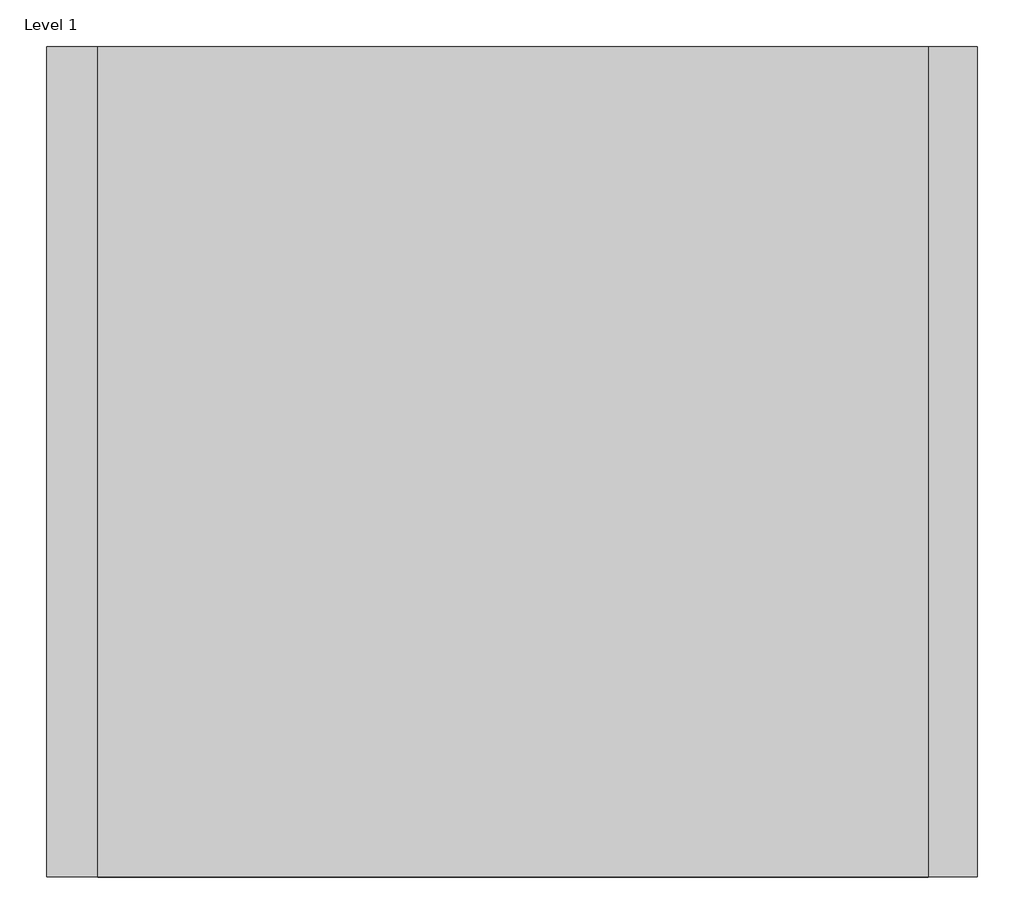
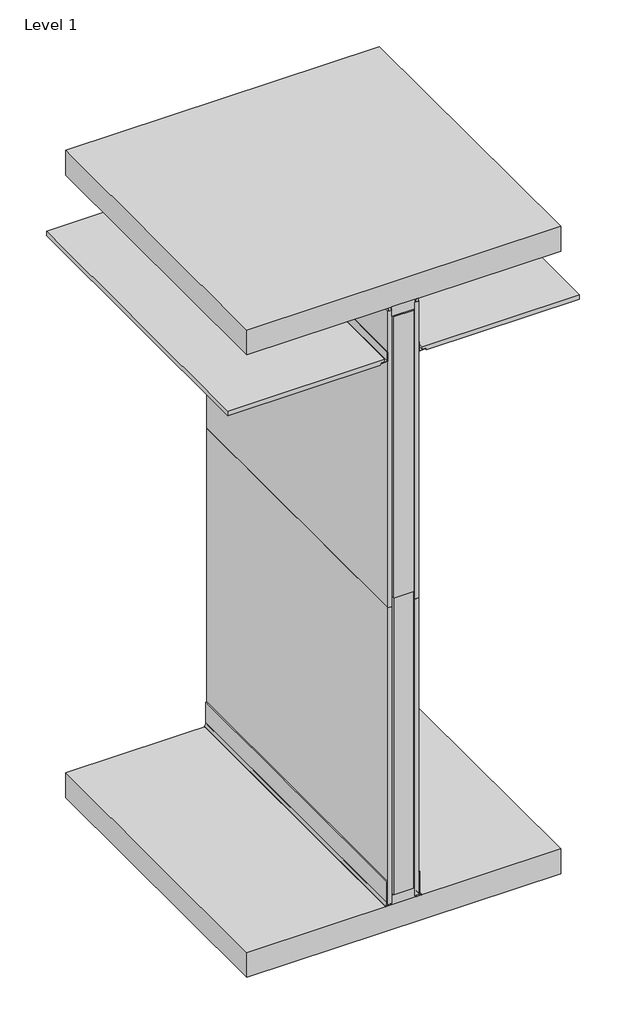
# One storey: 25 proxies.
"""IFC4 building model written with IfcOpenShell, lengths in millimetres."""

import ifcopenshell
import ifcopenshell.guid

model = None  # the IFC model being written
_history = None  # IfcOwnerHistory: only IFC2X3 demands one
_inside = {}  # id of a spatial element -> (the spatial element, [elements in it])
_under = {}  # id of a project, library or spatial element -> (it, [spatial elements below it])
_declared = {}  # id of a project -> (the project, [libraries it declares])
_typed = {}  # id of a type object -> (the type object, [elements of that type])
_made_of = {}  # id of a material, layer set ... -> (it, [elements and type objects made of it])


def new_model(schema):
    """Start an empty IFC model of exactly this schema.

    Asked for "IFC4X3", IfcOpenShell would pick the latest addendum, in which some entities
    have other attributes; the version numbers below select the first issue.
    IFC2X3 requires an IfcOwnerHistory on every rooted entity: one is made here for all.
    """
    global model, _history
    if schema == "IFC4X3":
        model = ifcopenshell.file(schema_version=(4, 3, 0, 0))
    else:
        model = ifcopenshell.file(schema=schema)
    _inside.clear()
    _under.clear()
    _declared.clear()
    _typed.clear()
    _made_of.clear()
    _history = None
    if model.schema == "IFC2X3":
        org = make("IfcOrganization", Name="unknown")
        user = make(
            "IfcPersonAndOrganization",
            ThePerson=make("IfcPerson", FamilyName="unknown"),
            TheOrganization=org,
        )
        app = make(
            "IfcApplication",
            ApplicationDeveloper=org,
            Version="unknown",
            ApplicationFullName="unknown",
            ApplicationIdentifier="unknown",
        )
        _history = make(
            "IfcOwnerHistory",
            OwningUser=user,
            OwningApplication=app,
            ChangeAction="ADDED",
            CreationDate=0,
        )
    return model


def make(cls, **values):
    """One entity of the class cls with the attributes given. An attribute that is None is left unset."""
    return model.create_entity(
        cls, **{name: value for name, value in values.items() if value is not None}
    )


def rooted(cls, **values):
    """An entity with a GlobalId (a new one), such as an element, a storey or a relation."""
    return make(cls, GlobalId=ifcopenshell.guid.new(), OwnerHistory=_history, **values)


def si_unit(unit_type, name, prefix=None):
    """IfcSIUnit, for example si_unit("LENGTHUNIT", "METRE", prefix="MILLI")."""
    return make("IfcSIUnit", UnitType=unit_type, Prefix=prefix, Name=name)


def assignment(units):
    """IfcUnitAssignment: the units of a project."""
    return None if units is None else make("IfcUnitAssignment", Units=units)


def point(xyz):
    """IfcCartesianPoint."""
    return None if xyz is None else make("IfcCartesianPoint", Coordinates=xyz)


def direction(xyz):
    """IfcDirection."""
    return None if xyz is None else make("IfcDirection", DirectionRatios=xyz)


def frame(location, z_axis=None, x_axis=None):
    """IfcAxis2Placement3D, a coordinate frame: its origin and axes. An axis left out is left unset."""
    return make(
        "IfcAxis2Placement3D",
        Location=point(location),
        Axis=direction(z_axis),
        RefDirection=direction(x_axis),
    )


def frame_2d(location, x_axis=None):
    """IfcAxis2Placement2D, a coordinate frame in the plane: its origin and x axis."""
    return make(
        "IfcAxis2Placement2D", Location=point(location), RefDirection=direction(x_axis)
    )


def origin():
    """The frame at (0, 0, 0) with its axes left unset."""
    return frame((0.0, 0.0, 0.0))


def place(relative_to, where):
    """IfcLocalPlacement: puts the frame where relative to a parent placement (None: the world)."""
    return make(
        "IfcLocalPlacement", PlacementRelTo=relative_to, RelativePlacement=where
    )


def context(
    kind, dimensions, precision=None, world=None, true_north=None, identifier=None
):
    """IfcGeometricRepresentationContext, for example the 3D "Model" context."""
    return make(
        "IfcGeometricRepresentationContext",
        ContextIdentifier=identifier,
        ContextType=kind,
        CoordinateSpaceDimension=dimensions,
        Precision=precision,
        WorldCoordinateSystem=world,
        TrueNorth=true_north,
    )


def project(units=None, contexts=None):
    """IfcProject with its units and contexts."""
    return rooted(
        "IfcProject",
        Name="project",
        RepresentationContexts=contexts,
        UnitsInContext=assignment(units),
    )


def spatial(cls, under=None, at=None, **own):
    """A site, building, storey or space (cls), placed at a placement, below another one or the project."""
    s = rooted(cls, ObjectPlacement=at, **own)
    if under is not None:
        _under.setdefault(under.id(), (under, []))[1].append(s)
    return s


def polyline(points):
    """IfcPolyline through the points."""
    return make("IfcPolyline", Points=[point(p) for p in points])


def circle_curve(where, radius):
    """IfcCircle in the frame where."""
    return make("IfcCircle", Position=where, Radius=radius)


def trimmed(basis, trim1, trim2, sense, master):
    """IfcTrimmedCurve: the piece of a basis curve between two trims."""
    return make(
        "IfcTrimmedCurve",
        BasisCurve=basis,
        Trim1=trim1,
        Trim2=trim2,
        SenseAgreement=sense,
        MasterRepresentation=master,
    )


def segment(curve, same_sense, transition):
    """IfcCompositeCurveSegment."""
    return make(
        "IfcCompositeCurveSegment",
        Transition=transition,
        SameSense=same_sense,
        ParentCurve=curve,
    )


def composite_curve(segments, self_intersect=None):
    """IfcCompositeCurve: segments joined end to end."""
    return make("IfcCompositeCurve", Segments=segments, SelfIntersect=self_intersect)


def outline(outer, holes=None, kind="AREA"):
    """IfcArbitraryClosedProfileDef: a profile drawn as a closed curve; with holes, ...WithVoids."""
    if holes is None:
        return make("IfcArbitraryClosedProfileDef", ProfileType=kind, OuterCurve=outer)
    return make(
        "IfcArbitraryProfileDefWithVoids",
        ProfileType=kind,
        OuterCurve=outer,
        InnerCurves=holes,
    )


def extrude(swept, where, along, depth):
    """IfcExtrudedAreaSolid: the profile swept, set in the frame where, extruded along a direction by depth."""
    return make(
        "IfcExtrudedAreaSolid",
        SweptArea=swept,
        Position=where,
        ExtrudedDirection=direction(along),
        Depth=depth,
    )


def shape(context_of_items, identifier, shape_type, items):
    """IfcShapeRepresentation: the items that make up one representation, for example the "Body"."""
    return make(
        "IfcShapeRepresentation",
        ContextOfItems=context_of_items,
        RepresentationIdentifier=identifier,
        RepresentationType=shape_type,
        Items=items,
    )


def source(mapping_origin, context_of_items, identifier, shape_type, items):
    """IfcRepresentationMap: a shape defined once, which mapped items show again and again."""
    return make(
        "IfcRepresentationMap",
        MappingOrigin=mapping_origin,
        MappedRepresentation=shape(context_of_items, identifier, shape_type, items),
    )


def transform(
    local_origin,
    x_axis=None,
    y_axis=None,
    z_axis=None,
    scale=None,
    scale2=None,
    scale3=None,
    uniform=True,
):
    """IfcCartesianTransformationOperator3D, or its non-uniform kind. x_axis, y_axis, z_axis: its Axis1, 2, 3."""
    if uniform:
        return make(
            "IfcCartesianTransformationOperator3D",
            Axis1=direction(x_axis),
            Axis2=direction(y_axis),
            LocalOrigin=point(local_origin),
            Scale=scale,
            Axis3=direction(z_axis),
        )
    return make(
        "IfcCartesianTransformationOperator3DnonUniform",
        Axis1=direction(x_axis),
        Axis2=direction(y_axis),
        LocalOrigin=point(local_origin),
        Scale=scale,
        Axis3=direction(z_axis),
        Scale2=scale2,
        Scale3=scale3,
    )


def mapped(mapping_source, mapping_target):
    """IfcMappedItem: shows the shape of a source again, moved by a transform."""
    return make(
        "IfcMappedItem", MappingSource=mapping_source, MappingTarget=mapping_target
    )


def made_of(thing, what):
    """Note that an element or type object is made of a material, layer set ...; save() writes the relation."""
    if what is not None:
        _made_of.setdefault(what.id(), (what, []))[1].append(thing)
    return thing


def element(
    cls,
    number,
    at=None,
    inside=None,
    cuts=None,
    type_object=None,
    material=None,
    context=None,
    identifier="Body",
    shape_type=None,
    held_by="IfcProductDefinitionShape",
    body=None,
    shapes=None,
    **own,
):
    """One element of the class cls, such as IfcWall. Its Tag is "e" and its number.

    at: its placement. inside: the storey or other place that contains it. cuts: it is an
    opening in that element (IfcRelVoidsElement). A single representation is given by context,
    identifier, shape_type and body (its items); several are given by shapes. held_by: the class
    of the entity that holds the representations. save() writes the other relations.
    """
    e = rooted(cls, Tag="e%d" % number, ObjectPlacement=at, **own)
    if body is not None:
        shapes = [shape(context, identifier, shape_type, body)]
    if shapes is not None:
        e.Representation = make(held_by, Representations=shapes)
    if inside is not None:
        _inside.setdefault(inside.id(), (inside, []))[1].append(e)
    if cuts is not None:
        rooted(
            "IfcRelVoidsElement", RelatingBuildingElement=cuts, RelatedOpeningElement=e
        )
    if type_object is not None:
        _typed.setdefault(type_object.id(), (type_object, []))[1].append(e)
    return made_of(e, material)


def aggregate(whole, parts):
    """IfcRelAggregates: a whole, such as a stair, and the parts it consists of."""
    return rooted("IfcRelAggregates", RelatingObject=whole, RelatedObjects=parts)


def save(model, path):
    """Write the relations noted so far, then the file.

    IfcRelAggregates (storeys below a building ...), IfcRelContainedInSpatialStructure (elements
    in a storey), IfcRelDefinesByType, IfcRelAssociatesMaterial and IfcRelDeclares: one each for
    every whole, place, type object, material and project.
    """
    for whole, parts in _under.values():
        aggregate(whole, parts)
    for where, things in _inside.values():
        rooted(
            "IfcRelContainedInSpatialStructure",
            RelatedElements=things,
            RelatingStructure=where,
        )
    for kind, things in _typed.values():
        rooted("IfcRelDefinesByType", RelatedObjects=things, RelatingType=kind)
    for what, things in _made_of.values():
        rooted("IfcRelAssociatesMaterial", RelatedObjects=things, RelatingMaterial=what)
    for by, libraries in _declared.values():
        rooted("IfcRelDeclares", RelatingContext=by, RelatedDefinitions=libraries)
    model.write(path)


def generic_models_70_generic_models_1_2fc778b0(model_context):
    return source(origin(), model_context, "Body", "SweptSolid", [
        extrude(outline(polyline([(51059.1296235, 0.0), (51043.2546235, 0.0), (51043.2546235, 1219.2), (51059.1296235, 1219.2), (51059.1296235, 0.0)])), frame((0.0, 0.0, 34.479891), z_axis=(0.0, 0.0, 1.0), x_axis=(1.0, 0.0, 0.0)), (0.0, 0.0, 1.0), 1219.2),
    ])


def generic_models_71_generic_models_1_dfea5cc7(model_context):
    return source(origin(), model_context, "Body", "SweptSolid", [
        extrude(outline(composite_curve([segment(trimmed(circle_curve(frame_2d((31.025412, 51021.9897405)), 4.3100275), [point((27.850412, 51019.075))], [point((34.200412, 51019.075))], True, "CARTESIAN"), True, "CONTINUOUS"), segment(polyline([(34.200412, 51019.075), (34.200412, 51009.55)]), True, "CONTINUOUS"), segment(trimmed(circle_curve(frame_2d((31.025412, 51012.4647405)), 4.3100275), [point((34.200412, 51009.55))], [point((27.850412, 51009.55))], False, "CARTESIAN"), True, "CONTINUOUS"), segment(polyline([(27.850412, 51009.55), (27.850412, 51019.075)]), True, "CONTINUOUS")], self_intersect=False)), frame((0.0, 0.0, 0.0), z_axis=(0.0, 1.0, 0.0), x_axis=(0.0, 0.0, 1.0)), (0.0, 0.0, 1.0), 1219.2),
    ])


def generic_models_72_generic_models_1_f511e09d(model_context):
    return source(origin(), model_context, "Body", "SweptSolid", [
        extrude(outline(polyline([(48561.625, 592.1375), (48472.725, 592.1375), (48472.725, 630.2375), (48561.625, 630.2375), (48561.625, 592.1375)])), frame((0.0, 0.0, 65.950412), z_axis=(0.0, 0.0, 1.0), x_axis=(1.0, 0.0, 0.0)), (0.0, 0.0, 1.0), 2381.25),
    ])


def generic_models_73_generic_models_1_7c4ccb31(model_context):
    return source(origin(), model_context, "Body", "SweptSolid", [
        extrude(outline(composite_curve([segment(polyline([(101.6, 51108.5310187), (15.4496307, 51108.5310187)]), True, "CONTINUOUS"), segment(trimmed(circle_curve(frame_2d((15.4496307, 51126.3707155)), 17.8396968), [point((15.4496307, 51108.5310187))], [point((0.0, 51117.4508671))], False, "CARTESIAN"), True, "CONTINUOUS"), segment(polyline([(0.0, 51117.4508671), (2.7496307, 51119.0383671)]), True, "CONTINUOUS"), segment(trimmed(circle_curve(frame_2d((15.4496307, 51126.3707155)), 14.6646968), [point((2.7496307, 51119.0383671))], [point((15.4496307, 51111.7060187))], True, "CARTESIAN"), True, "CONTINUOUS"), segment(polyline([(15.4496307, 51111.7060187), (99.5131982, 51111.7060187)]), True, "CONTINUOUS"), segment(trimmed(circle_curve(frame_2d((99.5131982, 51109.6192169)), 2.0868018), [point((99.5131982, 51111.7060187))], [point((101.6, 51109.6192169))], False, "CARTESIAN"), True, "CONTINUOUS"), segment(polyline([(101.6, 51109.6192169), (101.6, 51108.5310187)]), True, "CONTINUOUS")], self_intersect=False)), frame((0.0, 0.0, 0.0), z_axis=(0.0, 1.0, 0.0), x_axis=(0.0, 0.0, 1.0)), (0.0, 0.0, 1.0), 1219.2),
    ])


def generic_models_74_generic_models_1_1398e35e(model_context):
    return source(origin(), model_context, "Body", "SweptSolid", [
        extrude(outline(polyline([(48561.625, 0.0), (48472.725, 0.0), (48472.725, 1219.2), (48561.625, 1219.2), (48561.625, 0.0)])), frame((0.0, 0.0, 2447.200412), z_axis=(0.0, 0.0, 1.0), x_axis=(1.0, 0.0, 0.0)), (0.0, 0.0, 1.0), 38.1),
    ])


def generic_models_75_generic_models_1_c604be2e(model_context):
    return source(origin(), model_context, "Body", "SweptSolid", [
        extrude(outline(composite_curve([segment(trimmed(circle_curve(frame_2d((2472.600412, 51037.604481)), 8.620055), [point((2466.250412, 51031.775))], [point((2478.950412, 51031.775))], True, "CARTESIAN"), True, "CONTINUOUS"), segment(polyline([(2478.950412, 51031.775), (2478.950412, 51022.25)]), True, "CONTINUOUS"), segment(trimmed(circle_curve(frame_2d((2472.600412, 51028.079481)), 8.620055), [point((2478.950412, 51022.25))], [point((2466.250412, 51022.25))], False, "CARTESIAN"), True, "CONTINUOUS"), segment(polyline([(2466.250412, 51022.25), (2466.250412, 51031.775)]), True, "CONTINUOUS")], self_intersect=False)), frame((0.0, 0.0, 0.0), z_axis=(0.0, 1.0, 0.0), x_axis=(0.0, 0.0, 1.0)), (0.0, 0.0, 1.0), 1219.2),
    ])


def generic_models_77_generic_models_1_8544dbac(model_context):
    return source(origin(), model_context, "Body", "SweptSolid", [
        extrude(outline(polyline([(49128.3625, 0.0), (47909.1625, 0.0), (47909.1625, 1219.2), (49128.3625, 1219.2), (49128.3625, 0.0)])), frame((0.0, 0.0, 2485.300412), z_axis=(0.0, 0.0, 1.0), x_axis=(1.0, 0.0, 0.0)), (0.0, 0.0, 1.0), 101.6),
    ])


def generic_models_78_generic_models_1_faebf22d(model_context):
    return source(origin(), model_context, "Body", "SweptSolid", [
        extrude(outline(polyline([(51649.6572697, 0.0), (50430.4572697, 0.0), (50430.4572697, 1219.2), (51649.6572697, 1219.2), (51649.6572697, 0.0)])), frame((0.0, 0.0, -73.749588), z_axis=(0.0, 0.0, 1.0), x_axis=(1.0, 0.0, 0.0)), (0.0, 0.0, 1.0), 101.6),
    ])


def generic_models_79_generic_models_1_6d14886f(model_context):
    return source(origin(), model_context, "Body", "SweptSolid", [
        extrude(outline(polyline([(49776.0625, 0.0), (49699.8625, 0.0), (49699.8625, 1219.2), (49776.0625, 1219.2), (49776.0625, 0.0)])), frame((0.0, 0.0, 29.437912), z_axis=(0.0, 0.0, 1.0), x_axis=(1.0, 0.0, 0.0)), (0.0, 0.0, 1.0), 1219.2),
    ])


def generic_models_80_generic_models_1_8b1a960f(model_context):
    return source(origin(), model_context, "Body", "SweptSolid", [
        extrude(outline(polyline([(48556.8625, 0.0), (48480.6625, 0.0), (48480.6625, 1219.2), (48556.8625, 1219.2), (48556.8625, 0.0)])), frame((0.0, 0.0, 1264.512912), z_axis=(0.0, 0.0, 1.0), x_axis=(1.0, 0.0, 0.0)), (0.0, 0.0, 1.0), 1219.2),
    ])


def generic_models_81_generic_models_1_62cb9d11(model_context):
    return source(origin(), model_context, "Body", "SweptSolid", [
        extrude(outline(polyline([(2304.9709098, 49799.875), (2266.8709098, 49799.875), (2266.8709098, 49825.275), (2268.4584098, 49825.275), (2268.4584098, 49801.4625), (2304.9709098, 49801.4625), (2304.9709098, 49799.875)])), frame((0.0, 0.0, 0.0), z_axis=(0.0, 1.0, 0.0), x_axis=(0.0, 0.0, 1.0)), (0.0, 0.0, 1.0), 1219.2),
    ])


def generic_models_82_generic_models_1_f14c7ad8(model_context):
    return source(origin(), model_context, "Body", "SweptSolid", [
        extrude(outline(polyline([(2442.2225782, 49800.66875), (2442.2225782, 49799.875), (2439.6727146, 49799.875), (2437.6759782, 49723.675), (2435.6792418, 49799.875), (2433.1293782, 49799.875), (2433.1293782, 49800.66875), (2442.2225782, 49800.66875)])), frame((0.0, 565.15, 0.0), z_axis=(0.0, 1.0, 0.0), x_axis=(0.0, 0.0, 1.0)), (0.0, 0.0, 1.0), 12.7),
    ])


def generic_models_83_generic_models_1_66a13d42(model_context):
    return source(origin(), model_context, "Body", "SweptSolid", [
        extrude(outline(polyline([(2457.6119589, 49845.474547), (2457.6119589, 49854.567747), (2458.4057089, 49854.567747), (2458.4057089, 49852.0178834), (2534.6057089, 49850.021147), (2458.4057089, 49848.0244106), (2458.4057089, 49845.474547), (2457.6119589, 49845.474547)])), frame((0.0, 565.15, 0.0), z_axis=(0.0, 1.0, 0.0), x_axis=(0.0, 0.0, 1.0)), (0.0, 0.0, 1.0), 12.7),
    ])


def generic_models_84_generic_models_1_80fe95b7(model_context):
    return source(origin(), model_context, "Body", "SweptSolid", [
        extrude(outline(polyline([(48432.6703765, 0.0), (48416.7953765, 0.0), (48416.7953765, 1219.2), (48432.6703765, 1219.2), (48432.6703765, 0.0)])), frame((0.0, 0.0, 34.479891), z_axis=(0.0, 0.0, 1.0), x_axis=(1.0, 0.0, 0.0)), (0.0, 0.0, 1.0), 1219.2),
    ])


def generic_models_85_generic_models_1_c4fdf2dc(model_context):
    return source(origin(), model_context, "Body", "SweptSolid", [
        extrude(outline(composite_curve([segment(polyline([(27.850412, 48456.85), (27.850412, 48466.375)]), True, "CONTINUOUS"), segment(trimmed(circle_curve(frame_2d((31.025412, 48463.4602595)), 4.3100275), [point((27.850412, 48466.375))], [point((34.200412, 48466.375))], False, "CARTESIAN"), True, "CONTINUOUS"), segment(polyline([(34.200412, 48466.375), (34.200412, 48456.85)]), True, "CONTINUOUS"), segment(trimmed(circle_curve(frame_2d((31.025412, 48453.9352595)), 4.3100275), [point((34.200412, 48456.85))], [point((27.850412, 48456.85))], True, "CARTESIAN"), True, "CONTINUOUS")], self_intersect=False)), frame((0.0, 0.0, 0.0), z_axis=(0.0, 1.0, 0.0), x_axis=(0.0, 0.0, 1.0)), (0.0, 0.0, 1.0), 1219.2),
    ])


def generic_models_86_generic_models_1_e8e5dea3(model_context):
    return source(origin(), model_context, "Body", "SweptSolid", [
        extrude(outline(composite_curve([segment(polyline([(101.6, 48367.3939813), (101.6, 48366.3057831)]), True, "CONTINUOUS"), segment(trimmed(circle_curve(frame_2d((99.5131982, 48366.3057831)), 2.0868018), [point((101.6, 48366.3057831))], [point((99.5131982, 48364.2189813))], False, "CARTESIAN"), True, "CONTINUOUS"), segment(polyline([(99.5131982, 48364.2189813), (15.4496307, 48364.2189813)]), True, "CONTINUOUS"), segment(trimmed(circle_curve(frame_2d((15.4496307, 48349.5542845)), 14.6646968), [point((15.4496307, 48364.2189813))], [point((2.7496307, 48356.8866329))], True, "CARTESIAN"), True, "CONTINUOUS"), segment(polyline([(2.7496307, 48356.8866329), (0.0, 48358.4741329)]), True, "CONTINUOUS"), segment(trimmed(circle_curve(frame_2d((15.4496307, 48349.5542845)), 17.8396968), [point((0.0, 48358.4741329))], [point((15.4496307, 48367.3939813))], False, "CARTESIAN"), True, "CONTINUOUS"), segment(polyline([(15.4496307, 48367.3939813), (101.6, 48367.3939813)]), True, "CONTINUOUS")], self_intersect=False)), frame((0.0, 0.0, 0.0), z_axis=(0.0, 1.0, 0.0), x_axis=(0.0, 0.0, 1.0)), (0.0, 0.0, 1.0), 1219.2),
    ])


def generic_models_87_generic_models_1_0e45ed3c(model_context):
    return source(origin(), model_context, "Body", "SweptSolid", [
        extrude(outline(composite_curve([segment(polyline([(2466.250412, 48444.15), (2466.250412, 48453.675)]), True, "CONTINUOUS"), segment(trimmed(circle_curve(frame_2d((2472.600412, 48447.845519)), 8.620055), [point((2466.250412, 48453.675))], [point((2478.950412, 48453.675))], False, "CARTESIAN"), True, "CONTINUOUS"), segment(polyline([(2478.950412, 48453.675), (2478.950412, 48444.15)]), True, "CONTINUOUS"), segment(trimmed(circle_curve(frame_2d((2472.600412, 48438.320519)), 8.620055), [point((2478.950412, 48444.15))], [point((2466.250412, 48444.15))], True, "CARTESIAN"), True, "CONTINUOUS")], self_intersect=False)), frame((0.0, 0.0, 0.0), z_axis=(0.0, 1.0, 0.0), x_axis=(0.0, 0.0, 1.0)), (0.0, 0.0, 1.0), 1219.2),
    ])


def generic_models_89_generic_models_1_217c0eea(model_context):
    return source(origin(), model_context, "Body", "SweptSolid", [
        extrude(outline(polyline([(2304.9709098, 49676.05), (2304.9709098, 49674.4625), (2268.4584098, 49674.4625), (2268.4584098, 49650.65), (2266.8709098, 49650.65), (2266.8709098, 49676.05), (2304.9709098, 49676.05)])), frame((0.0, 0.0, 0.0), z_axis=(0.0, 1.0, 0.0), x_axis=(0.0, 0.0, 1.0)), (0.0, 0.0, 1.0), 1219.2),
    ])


def generic_models_90_generic_models_1_e41f1d4b(model_context):
    return source(origin(), model_context, "Body", "SweptSolid", [
        extrude(outline(polyline([(2281.1808399, 49662.5798593), (2281.1808399, 49052.9798593), (2262.1308399, 49052.9798593), (2262.1308399, 49646.9908455), (2270.0683399, 49649.8798593), (2270.0683399, 49662.5798593), (2281.1808399, 49662.5798593)])), frame((0.0, 0.0, 0.0), z_axis=(0.0, 1.0, 0.0), x_axis=(0.0, 0.0, 1.0)), (0.0, 0.0, 1.0), 1219.2),
    ])


def generic_models_91_generic_models_1_b13b52c1(model_context):
    return source(origin(), model_context, "Body", "SweptSolid", [
        extrude(outline(polyline([(2442.2225782, 49675.25625), (2433.1293782, 49675.25625), (2433.1293782, 49676.05), (2435.6792418, 49676.05), (2437.6759782, 49752.25), (2439.6727146, 49676.05), (2442.2225782, 49676.05), (2442.2225782, 49675.25625)])), frame((0.0, 565.15, 0.0), z_axis=(0.0, 1.0, 0.0), x_axis=(0.0, 0.0, 1.0)), (0.0, 0.0, 1.0), 12.7),
    ])


def generic_models_92_generic_models_1_05829357(model_context):
    return source(origin(), model_context, "Body", "SweptSolid", [
        extrude(outline(polyline([(67.537912, 48511.0409), (66.744162, 48511.0409), (66.744162, 48513.5907636), (-9.455838, 48515.5875), (66.744162, 48517.5842364), (66.744162, 48520.1341), (67.537912, 48520.1341), (67.537912, 48511.0409)])), frame((0.0, 565.15, 0.0), z_axis=(0.0, 1.0, 0.0), x_axis=(0.0, 0.0, 1.0)), (0.0, 0.0, 1.0), 12.7),
    ])


def generic_models_93_generic_models_1_4e4062ca(model_context):
    return source(origin(), model_context, "Body", "SweptSolid", [
        extrude(outline(polyline([(2281.1808399, 49813.3451407), (2270.0683399, 49813.3451407), (2270.0683399, 49826.0451407), (2262.1308399, 49828.9341545), (2262.1308399, 50422.9451407), (2281.1808399, 50422.9451407), (2281.1808399, 49813.3451407)])), frame((0.0, 0.0, 0.0), z_axis=(0.0, 1.0, 0.0), x_axis=(0.0, 0.0, 1.0)), (0.0, 0.0, 1.0), 1219.2),
    ])


model = new_model("IFC4")

# Units and contexts
model_context = context("Model", 3, world=origin())
ifc_project = project(units=[si_unit("LENGTHUNIT", "METRE", prefix="MILLI")], contexts=[model_context])

# Site, building, storey
site = spatial("IfcSite", under=ifc_project)
building = spatial("IfcBuilding", under=site)
storey = spatial("IfcBuildingStorey", under=building, Name="Level 1", Elevation=266395.2)

# Proxies
placement = place(None, origin())
generic_models_70_generic_models_1_shape = generic_models_70_generic_models_1_2fc778b0(model_context)
element("IfcBuildingElementProxy", 1, Name="Generic Models 70 : Generic Models 1", ObjectType="Generic Models 70 : Generic Models 1", at=placement, inside=storey, context=model_context, shape_type="MappedRepresentation", body=[
    mapped(generic_models_70_generic_models_1_shape, transform((-2481.6296235, 0.0, -0.279479), x_axis=(1.0, 0.0, 0.0), y_axis=(0.0, 1.0, 0.0), z_axis=(0.0, 0.0, 1.0))),
])
generic_models_71_generic_models_1_shape = generic_models_71_generic_models_1_dfea5cc7(model_context)
element("IfcBuildingElementProxy", 2, Name="Generic Models 71 : Generic Models 1", ObjectType="Generic Models 71 : Generic Models 1", at=placement, inside=storey, context=model_context, shape_type="MappedRepresentation", body=[
    mapped(generic_models_71_generic_models_1_shape, transform((-2441.575, 0.0, 0.0), x_axis=(1.0, 0.0, 0.0), y_axis=(0.0, 1.0, 0.0), z_axis=(0.0, 0.0, 1.0))),
])
generic_models_72_generic_models_1_shape = generic_models_72_generic_models_1_f511e09d(model_context)
element("IfcBuildingElementProxy", 3, Name="Generic Models 72 : Generic Models 1", ObjectType="Generic Models 72 : Generic Models 1", at=placement, inside=storey, context=model_context, shape_type="MappedRepresentation", body=[
    mapped(generic_models_72_generic_models_1_shape, transform((0.0, 0.0, 0.0), x_axis=(1.0, 0.0, 0.0), y_axis=(0.0, 1.0, 0.0), z_axis=(0.0, 0.0, 1.0))),
])
generic_models_73_generic_models_1_shape = generic_models_73_generic_models_1_7c4ccb31(model_context)
element("IfcBuildingElementProxy", 4, Name="Generic Models 73 : Generic Models 1", ObjectType="Generic Models 73 : Generic Models 1", at=placement, inside=storey, context=model_context, shape_type="MappedRepresentation", body=[
    mapped(generic_models_73_generic_models_1_shape, transform((-2531.0310187, 0.0, 27.850412), x_axis=(1.0, 0.0, 0.0), y_axis=(0.0, 1.0, 0.0), z_axis=(0.0, 0.0, 1.0))),
])
generic_models_74_generic_models_1_shape = generic_models_74_generic_models_1_1398e35e(model_context)
element("IfcBuildingElementProxy", 5, Name="Generic Models 74 : Generic Models 1", ObjectType="Generic Models 74 : Generic Models 1", at=placement, inside=storey, context=model_context, shape_type="MappedRepresentation", body=[
    mapped(generic_models_74_generic_models_1_shape, transform((0.0, 0.0, 0.0), x_axis=(1.0, 0.0, 0.0), y_axis=(0.0, 1.0, 0.0), z_axis=(0.0, 0.0, 1.0))),
])
generic_models_75_generic_models_1_shape = generic_models_75_generic_models_1_c604be2e(model_context)
element("IfcBuildingElementProxy", 6, Name="Generic Models 75 : Generic Models 1", ObjectType="Generic Models 75 : Generic Models 1", at=placement, inside=storey, context=model_context, shape_type="MappedRepresentation", body=[
    mapped(generic_models_75_generic_models_1_shape, transform((-2454.275, 0.0, 6.35), x_axis=(1.0, 0.0, 0.0), y_axis=(0.0, 1.0, 0.0), z_axis=(0.0, 0.0, 1.0))),
])
element("IfcBuildingElementProxy", 7, Name="Generic Models 76 : Generic Models 1", ObjectType="Generic Models 76 : Generic Models 1", at=placement, inside=storey, context=model_context, shape_type="MappedRepresentation", body=[
    mapped(generic_models_70_generic_models_1_shape, transform((-2481.6296235, 0.0, 1218.920521), x_axis=(1.0, 0.0, 0.0), y_axis=(0.0, 1.0, 0.0), z_axis=(0.0, 0.0, 1.0))),
])
generic_models_77_generic_models_1_shape = generic_models_77_generic_models_1_8544dbac(model_context)
element("IfcBuildingElementProxy", 8, Name="Generic Models 77 : Generic Models 1", ObjectType="Generic Models 77 : Generic Models 1", at=placement, inside=storey, context=model_context, shape_type="MappedRepresentation", body=[
    mapped(generic_models_77_generic_models_1_shape, transform((0.0, 0.0, 0.0), x_axis=(1.0, 0.0, 0.0), y_axis=(0.0, 1.0, 0.0), z_axis=(0.0, 0.0, 1.0))),
])
generic_models_78_generic_models_1_shape = generic_models_78_generic_models_1_faebf22d(model_context)
element("IfcBuildingElementProxy", 9, Name="Generic Models 78 : Generic Models 1", ObjectType="Generic Models 78 : Generic Models 1", at=placement, inside=storey, context=model_context, shape_type="MappedRepresentation", body=[
    mapped(generic_models_78_generic_models_1_shape, transform((-2521.2947697, 0.0, 0.0), x_axis=(1.0, 0.0, 0.0), y_axis=(0.0, 1.0, 0.0), z_axis=(0.0, 0.0, 1.0))),
])
generic_models_79_generic_models_1_shape = generic_models_79_generic_models_1_6d14886f(model_context)
element("IfcBuildingElementProxy", 10, Name="Generic Models 79 : Generic Models 1", ObjectType="Generic Models 79 : Generic Models 1", at=placement, inside=storey, context=model_context, shape_type="MappedRepresentation", body=[
    mapped(generic_models_79_generic_models_1_shape, transform((-1220.7875, 0.0, 36.5125), x_axis=(1.0, 0.0, 0.0), y_axis=(0.0, 1.0, 0.0), z_axis=(0.0, 0.0, 1.0))),
])
generic_models_80_generic_models_1_shape = generic_models_80_generic_models_1_8b1a960f(model_context)
element("IfcBuildingElementProxy", 11, Name="Generic Models 80 : Generic Models 1", ObjectType="Generic Models 80 : Generic Models 1", at=placement, inside=storey, context=model_context, shape_type="MappedRepresentation", body=[
    mapped(generic_models_80_generic_models_1_shape, transform((0.0, 0.0, -41.275), x_axis=(1.0, 0.0, 0.0), y_axis=(0.0, 1.0, 0.0), z_axis=(0.0, 0.0, 1.0))),
])
generic_models_81_generic_models_1_shape = generic_models_81_generic_models_1_62cb9d11(model_context)
element("IfcBuildingElementProxy", 12, Name="Generic Models 81 : Generic Models 1", ObjectType="Generic Models 81 : Generic Models 1", at=placement, inside=storey, context=model_context, shape_type="MappedRepresentation", body=[
    mapped(generic_models_81_generic_models_1_shape, transform((-1222.375, 0.0, 0.0), x_axis=(1.0, 0.0, 0.0), y_axis=(0.0, 1.0, 0.0), z_axis=(0.0, 0.0, 1.0))),
])
generic_models_82_generic_models_1_shape = generic_models_82_generic_models_1_f14c7ad8(model_context)
element("IfcBuildingElementProxy", 13, Name="Generic Models 82 : Generic Models 1", ObjectType="Generic Models 82 : Generic Models 1", at=placement, inside=storey, context=model_context, shape_type="MappedRepresentation", body=[
    mapped(generic_models_82_generic_models_1_shape, transform((-1222.375, 0.0, 17.4619338), x_axis=(1.0, 0.0, 0.0), y_axis=(0.0, 1.0, 0.0), z_axis=(0.0, 0.0, 1.0))),
])
generic_models_83_generic_models_1_shape = generic_models_83_generic_models_1_66a13d42(model_context)
element("IfcBuildingElementProxy", 14, Name="Generic Models 83 : Generic Models 1", ObjectType="Generic Models 83 : Generic Models 1", at=placement, inside=storey, context=model_context, shape_type="MappedRepresentation", body=[
    mapped(generic_models_83_generic_models_1_shape, transform((-1334.433647, 0.0, 25.3072031), x_axis=(1.0, 0.0, 0.0), y_axis=(0.0, 1.0, 0.0), z_axis=(0.0, 0.0, 1.0))),
])
generic_models_84_generic_models_1_shape = generic_models_84_generic_models_1_80fe95b7(model_context)
element("IfcBuildingElementProxy", 15, Name="Generic Models 84 : Generic Models 1", ObjectType="Generic Models 84 : Generic Models 1", at=placement, inside=storey, context=model_context, shape_type="MappedRepresentation", body=[
    mapped(generic_models_84_generic_models_1_shape, transform((40.0546235, 0.0, -0.279479), x_axis=(1.0, 0.0, 0.0), y_axis=(0.0, 1.0, 0.0), z_axis=(0.0, 0.0, 1.0))),
])
generic_models_85_generic_models_1_shape = generic_models_85_generic_models_1_c4fdf2dc(model_context)
element("IfcBuildingElementProxy", 16, Name="Generic Models 85 : Generic Models 1", ObjectType="Generic Models 85 : Generic Models 1", at=placement, inside=storey, context=model_context, shape_type="MappedRepresentation", body=[
    mapped(generic_models_85_generic_models_1_shape, transform((0.0, 0.0, 0.0), x_axis=(1.0, 0.0, 0.0), y_axis=(0.0, 1.0, 0.0), z_axis=(0.0, 0.0, 1.0))),
])
generic_models_86_generic_models_1_shape = generic_models_86_generic_models_1_e8e5dea3(model_context)
element("IfcBuildingElementProxy", 17, Name="Generic Models 86 : Generic Models 1", ObjectType="Generic Models 86 : Generic Models 1", at=placement, inside=storey, context=model_context, shape_type="MappedRepresentation", body=[
    mapped(generic_models_86_generic_models_1_shape, transform((89.4560187, 0.0, 27.850412), x_axis=(1.0, 0.0, 0.0), y_axis=(0.0, 1.0, 0.0), z_axis=(0.0, 0.0, 1.0))),
])
generic_models_87_generic_models_1_shape = generic_models_87_generic_models_1_0e45ed3c(model_context)
element("IfcBuildingElementProxy", 18, Name="Generic Models 87 : Generic Models 1", ObjectType="Generic Models 87 : Generic Models 1", at=placement, inside=storey, context=model_context, shape_type="MappedRepresentation", body=[
    mapped(generic_models_87_generic_models_1_shape, transform((12.7, 0.0, 6.35), x_axis=(1.0, 0.0, 0.0), y_axis=(0.0, 1.0, 0.0), z_axis=(0.0, 0.0, 1.0))),
])
element("IfcBuildingElementProxy", 19, Name="Generic Models 88 : Generic Models 1", ObjectType="Generic Models 88 : Generic Models 1", at=placement, inside=storey, context=model_context, shape_type="MappedRepresentation", body=[
    mapped(generic_models_84_generic_models_1_shape, transform((40.0546235, 0.0, 1218.920521), x_axis=(1.0, 0.0, 0.0), y_axis=(0.0, 1.0, 0.0), z_axis=(0.0, 0.0, 1.0))),
])
generic_models_89_generic_models_1_shape = generic_models_89_generic_models_1_217c0eea(model_context)
element("IfcBuildingElementProxy", 20, Name="Generic Models 89 : Generic Models 1", ObjectType="Generic Models 89 : Generic Models 1", at=placement, inside=storey, context=model_context, shape_type="MappedRepresentation", body=[
    mapped(generic_models_89_generic_models_1_shape, transform((-1219.2, 0.0, 0.0), x_axis=(1.0, 0.0, 0.0), y_axis=(0.0, 1.0, 0.0), z_axis=(0.0, 0.0, 1.0))),
])
generic_models_90_generic_models_1_shape = generic_models_90_generic_models_1_e41f1d4b(model_context)
element("IfcBuildingElementProxy", 21, Name="Generic Models 90 : Generic Models 1", ObjectType="Generic Models 90 : Generic Models 1", at=placement, inside=storey, context=model_context, shape_type="MappedRepresentation", body=[
    mapped(generic_models_90_generic_models_1_shape, transform((-1219.2, 0.0, 0.0), x_axis=(1.0, 0.0, 0.0), y_axis=(0.0, 1.0, 0.0), z_axis=(0.0, 0.0, 1.0))),
])
generic_models_91_generic_models_1_shape = generic_models_91_generic_models_1_b13b52c1(model_context)
element("IfcBuildingElementProxy", 22, Name="Generic Models 91 : Generic Models 1", ObjectType="Generic Models 91 : Generic Models 1", at=placement, inside=storey, context=model_context, shape_type="MappedRepresentation", body=[
    mapped(generic_models_91_generic_models_1_shape, transform((-1219.2, 0.0, 22.2244338), x_axis=(1.0, 0.0, 0.0), y_axis=(0.0, 1.0, 0.0), z_axis=(0.0, 0.0, 1.0))),
])
generic_models_92_generic_models_1_shape = generic_models_92_generic_models_1_05829357(model_context)
element("IfcBuildingElementProxy", 23, Name="Generic Models 92 : Generic Models 1", ObjectType="Generic Models 92 : Generic Models 1", at=placement, inside=storey, context=model_context, shape_type="MappedRepresentation", body=[
    mapped(generic_models_92_generic_models_1_shape, transform((0.0, 0.0, 0.0), x_axis=(1.0, 0.0, 0.0), y_axis=(0.0, 1.0, 0.0), z_axis=(0.0, 0.0, 1.0))),
])
generic_models_93_generic_models_1_shape = generic_models_93_generic_models_1_4e4062ca(model_context)
element("IfcBuildingElementProxy", 24, Name="Generic Models 93 : Generic Models 1", ObjectType="Generic Models 93 : Generic Models 1", at=placement, inside=storey, context=model_context, shape_type="MappedRepresentation", body=[
    mapped(generic_models_93_generic_models_1_shape, transform((-1222.375, 0.0, 0.0), x_axis=(1.0, 0.0, 0.0), y_axis=(0.0, 1.0, 0.0), z_axis=(0.0, 0.0, 1.0))),
])
element("IfcBuildingElementProxy", 25, Name="Generic Models 94 : Generic Models 1", ObjectType="Generic Models 94 : Generic Models 1", at=placement, inside=storey, context=model_context, shape_type="MappedRepresentation", body=[
    mapped(generic_models_74_generic_models_1_shape, transform((0.0, 0.0, -2419.35), x_axis=(1.0, 0.0, 0.0), y_axis=(0.0, 1.0, 0.0), z_axis=(0.0, 0.0, 1.0))),
])

save(model, "model.ifc")

# Revit data of these elements
# Project information
#   Project Issue Date = "Issue Date"
#   Project Status = "Project Status"
#   Client Name = "Owner"
#   Project Address = "640 West Main Street, Lake Geneva, WI 53147"
#   Project Name = "The Downtowner"
#   Project Number = "Project Number"
# Element 1 (IfcBuildingElementProxy, "Generic Models 70 : Generic Models 1")
#   Phase Created = New Construction
#   Materials on its faces: "5/8\" GYP. BD"
# Element 2 (IfcBuildingElementProxy, "Generic Models 71 : Generic Models 1")
#   Phase Created = New Construction
#   Materials on its faces: "ACOUSTICAL SEALANT"
# Element 3 (IfcBuildingElementProxy, "Generic Models 72 : Generic Models 1")
#   Phase Created = New Construction
#   Materials on its faces: "METAL STUDS (MATCH EXISTING SIZE/GAUGE/SPACING)"
# Element 4 (IfcBuildingElementProxy, "Generic Models 73 : Generic Models 1")
#   Phase Created = New Construction
#   Materials on its faces: "BASE AS SCHEDULED"
# Element 5 (IfcBuildingElementProxy, "Generic Models 74 : Generic Models 1")
#   Phase Created = New Construction
#   Materials on its faces: "2X4 WOOD STUDS"
# Element 6 (IfcBuildingElementProxy, "Generic Models 75 : Generic Models 1")
#   Phase Created = New Construction
#   Materials on its faces: "ACOUSTICAL SEALANT"
# Element 7 (IfcBuildingElementProxy, "Generic Models 76 : Generic Models 1")
#   Phase Created = New Construction
#   Materials on its faces: "5/8\" GYP. BD"
# Element 8 (IfcBuildingElementProxy, "Generic Models 77 : Generic Models 1")
#   Phase Created = New Construction
#   Materials on its faces: "UNDERSIDE OF STRUCTURE"
# Element 9 (IfcBuildingElementProxy, "Generic Models 78 : Generic Models 1")
#   Phase Created = New Construction
#   Materials on its faces: "STRUCTURAL FLOOR"
# Element 10 (IfcBuildingElementProxy, "Generic Models 79 : Generic Models 1")
#   Phase Created = New Construction
#   Materials on its faces: "SOUND BATT. INSULATION (THICKNESS TO MATCH WALL DEPTH)"
# Element 11 (IfcBuildingElementProxy, "Generic Models 80 : Generic Models 1")
#   Phase Created = New Construction
#   Materials on its faces: "SOUND BATT. INSULATION (THICKNESS TO MATCH WALL DEPTH)"
# Element 12 (IfcBuildingElementProxy, "Generic Models 81 : Generic Models 1")
#   Phase Created = New Construction
#   Materials on its faces: "CEILING TRACK AS SCHEDULED"
# Element 13 (IfcBuildingElementProxy, "Generic Models 82 : Generic Models 1")
#   Phase Created = New Construction
#   Materials on its faces: "ATTACH GYPSUM BOARD TO STUDS AND NOT TO TOP TRACK"
# Element 14 (IfcBuildingElementProxy, "Generic Models 83 : Generic Models 1")
#   Phase Created = New Construction
#   Materials on its faces: "ATTACH GYPSUM BOARD TO STUDS AND NOT TO TOP TRACK"
# Element 15 (IfcBuildingElementProxy, "Generic Models 84 : Generic Models 1")
#   Phase Created = New Construction
#   Materials on its faces: "5/8\" GYP. BD"
# Element 16 (IfcBuildingElementProxy, "Generic Models 85 : Generic Models 1")
#   Phase Created = New Construction
#   Materials on its faces: "ACOUSTICAL SEALANT"
# Element 17 (IfcBuildingElementProxy, "Generic Models 86 : Generic Models 1")
#   Phase Created = New Construction
#   Materials on its faces: "BASE AS SCHEDULED"
# Element 18 (IfcBuildingElementProxy, "Generic Models 87 : Generic Models 1")
#   Phase Created = New Construction
#   Materials on its faces: "ACOUSTICAL SEALANT"
# Element 19 (IfcBuildingElementProxy, "Generic Models 88 : Generic Models 1")
#   Phase Created = New Construction
#   Materials on its faces: "5/8\" GYP. BD"
# Element 20 (IfcBuildingElementProxy, "Generic Models 89 : Generic Models 1")
#   Phase Created = New Construction
#   Materials on its faces: "CEILING TRACK AS SCHEDULED"
# Element 21 (IfcBuildingElementProxy, "Generic Models 90 : Generic Models 1")
#   Phase Created = New Construction
#   Materials on its faces: "CEILING AS SCHEDULED"
# Element 22 (IfcBuildingElementProxy, "Generic Models 91 : Generic Models 1")
#   Phase Created = New Construction
#   Materials on its faces: "ATTACH GYPSUM BOARD TO STUDS AND NOT TO TOP TRACK"
# Element 23 (IfcBuildingElementProxy, "Generic Models 92 : Generic Models 1")
#   Phase Created = New Construction
#   Materials on its faces: "ATTACH GYPSUM BOARD TO STUDS AND NOT TO TOP TRACK"
# Element 24 (IfcBuildingElementProxy, "Generic Models 93 : Generic Models 1")
#   Phase Created = New Construction
#   Materials on its faces: "CEILING AS SCHEDULED"
# Element 25 (IfcBuildingElementProxy, "Generic Models 94 : Generic Models 1")
#   Phase Created = New Construction
#   Materials on its faces: "2X4 WOOD STUDS"
# Materials
#   "5/8\" GYP. BD": class "Generic", colour RGB 136 135 132, transparency 0, Description = "Gypsum Wall Board", Cost = 0
#   "ACOUSTICAL SEALANT": class "Unassigned", colour RGB 120 120 120, transparency 0, Cost = 0
#   "METAL STUDS (MATCH EXISTING SIZE/GAUGE/SPACING)": class "Unassigned", colour RGB 210 209 208, transparency 0, Keynote = "M05121300.02", Cost = 0
#   "BASE AS SCHEDULED": class "Generic", colour RGB 120 120 120, transparency 0, Cost = 0
#   "2X4 WOOD STUDS": class "Wood", colour RGB 144 113 62, transparency 0, Description = "Pinus Echinata", Cost = 0
#   "UNDERSIDE OF STRUCTURE": class "Concrete", colour RGB 115 116 108, transparency 0, Description = "Lightweight concrete", Cost = 0
#   "STRUCTURAL FLOOR": class "Concrete", colour RGB 115 116 108, transparency 0, Description = "Lightweight concrete", Cost = 0
#   "SOUND BATT. INSULATION (THICKNESS TO MATCH WALL DEPTH)": class "Unassigned", colour RGB 255 255 255, transparency 0, Cost = 0
#   "CEILING TRACK AS SCHEDULED": class "Unassigned", colour RGB 210 209 208, transparency 0, Keynote = "M05121300.02", Cost = 0
#   "ATTACH GYPSUM BOARD TO STUDS AND NOT TO TOP TRACK": class "Generic", colour RGB 48 48 48, transparency 0, Cost = 0
#   "CEILING AS SCHEDULED": class "Generic", colour RGB 255 255 255, transparency 0, Cost = 0
